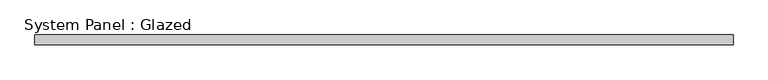
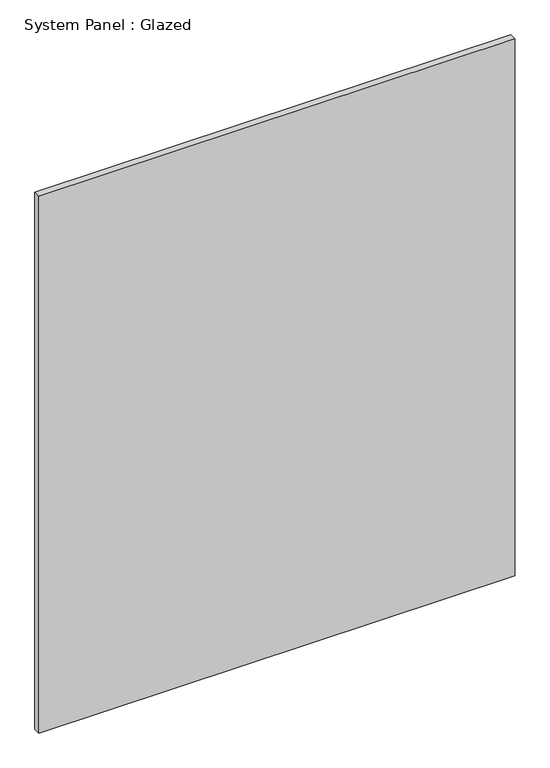
"""IFC4 building model written with IfcOpenShell, lengths in millimetres: plate geometry, System Panel : Glazed."""

from ifc_helpers import new_model, si_unit, origin, origin_with_axes, place, context, project, spatial, polyline, outline, extrude, source, transform, mapped, element, save


def system_panel_glazed_e1602509(model_context):
    return source(origin(), model_context, "Body", "SweptSolid", [
        extrude(outline(polyline([(891.0, -49.5), (-891.0, -49.5), (-891.0, -24.5), (891.0, -24.5), (891.0, -49.5)])), origin_with_axes(), (0.0, 0.0, 1.0), 2125.0),
    ])


if __name__ == "__main__":
    model = new_model("IFC4")
    model_context = context("Model", 3, world=origin())
    ifc_project = project(units=[si_unit("LENGTHUNIT", "METRE", prefix="MILLI")], contexts=[model_context])
    site = spatial("IfcSite", under=ifc_project)
    building = spatial("IfcBuilding", under=site)
    placement = place(None, origin())
    system_panel_glazed_shape = system_panel_glazed_e1602509(model_context)
    element("IfcPlate", 1, ObjectType="System Panel : Glazed", at=placement, inside=building, context=model_context, shape_type="MappedRepresentation", body=[
        mapped(system_panel_glazed_shape, transform((0.0, 0.0, 0.0), x_axis=(1.0, 0.0, 0.0), y_axis=(0.0, 1.0, 0.0), z_axis=(0.0, 0.0, 1.0))),
    ])
    save(model, "model.ifc")

# Revit data of these elements
# Type "System Panel : Glazed"
#   Keynote = "H11"
#   Construction Type Id = "GSP4R"
#   Analytic Construction = "1/8 in Pilkington single glazing"
#   Visual Light Transmittance = 0.9
#   Solar Heat Gain Coefficient = 0.86
#   Heat Transfer Coefficient (U) = 6.7069 W/(m²·K)
# Element 1 (IfcPlate, "System Panel : Glazed")
#   Materials on its faces: "Glass"
# Materials
#   "Glass": class "Glass", colour RGB 0 128 192, transparency 0.9, Description = "Soda Lime Glass", Cost = 0
